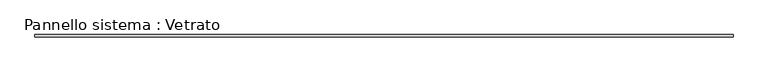
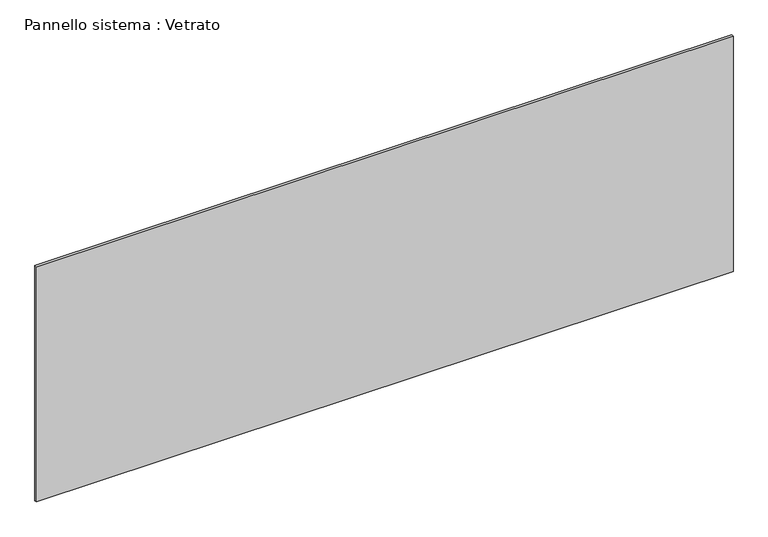
"""IFC4 building model written with IfcOpenShell, lengths in millimetres: plate geometry, Pannello sistema : Vetrato."""

from ifc_helpers import new_model, si_unit, origin, origin_with_axes, place, context, project, spatial, polyline, outline, extrude, source, transform, mapped, element, save


def pannello_sistema_vetrato_29ff3466(model_context):
    return source(origin(), model_context, "Body", "SweptSolid", [
        extrude(outline(polyline([(4200.0000001, -15.0), (-4200.0000001, -15.0), (-4200.0000001, 15.0), (4200.0000001, 15.0), (4200.0000001, -15.0)])), origin_with_axes(), (0.0, 0.0, 1.0), 3000.0),
    ])


if __name__ == "__main__":
    model = new_model("IFC4")
    model_context = context("Model", 3, world=origin())
    ifc_project = project(units=[si_unit("LENGTHUNIT", "METRE", prefix="MILLI")], contexts=[model_context])
    site = spatial("IfcSite", under=ifc_project)
    building = spatial("IfcBuilding", under=site)
    placement = place(None, origin())
    pannello_sistema_vetrato_shape = pannello_sistema_vetrato_29ff3466(model_context)
    element("IfcPlate", 1, ObjectType="Pannello sistema : Vetrato", at=placement, inside=building, context=model_context, shape_type="MappedRepresentation", body=[
        mapped(pannello_sistema_vetrato_shape, transform((0.0, 0.0, 0.0), x_axis=(1.0, 0.0, 0.0), y_axis=(0.0, 1.0, 0.0), z_axis=(0.0, 0.0, 1.0))),
    ])
    save(model, "model.ifc")

# Revit data of these elements
# Type "Pannello sistema : Vetrato"
#   Construction Type Id = "GSP4R"
#   Analytic Construction = "Vetrata singola Pilkington 1/8 in"
#   Visual Light Transmittance = 0.9
#   Solar Heat Gain Coefficient = 0.86
#   Heat Transfer Coefficient (U) = 6.7069 W/(m²·K)
# Element 1 (IfcPlate, "Pannello sistema : Vetrato")
#   Materials on its faces: "Default - Vetro"
# Materials
#   "Default - Vetro": class "Vetro", colour RGB 208 208 208, transparency 0.7, Cost = 0
